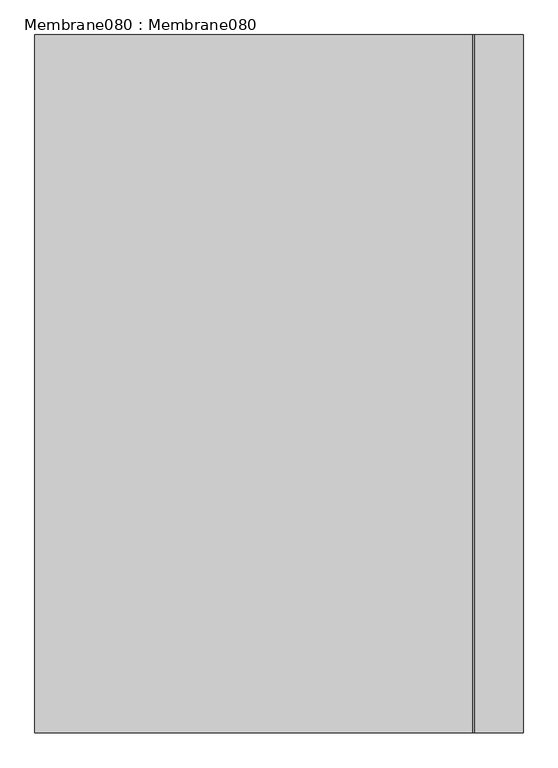
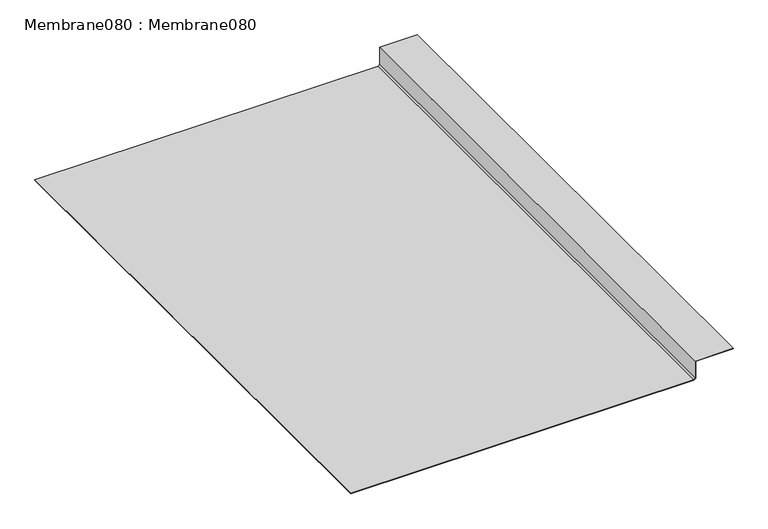
"""IFC4 building model written with IfcOpenShell, lengths in millimetres: proxy geometry, Membrane080 : Membrane080."""

from ifc_helpers import new_model, si_unit, frame, origin, place, context, project, spatial, polyline, outline, extrude, source, transform, mapped, element, save


def membrane080_membrane080_50d92a24(model_context):
    return source(origin(), model_context, "Body", "SweptSolid", [
        extrude(outline(polyline([(36549.109375, -1995.5294189), (36549.109375, -2134.3322754), (36483.4346119, -2134.3322754), (36478.390625, -2139.6929064), (36478.390625, -3395.3427853), (36476.390625, -3395.3427853), (36476.390625, -2138.8999023), (36482.5703125, -2132.3322754), (36547.109375, -2132.3322754), (36547.109375, -1995.5294189), (36549.109375, -1995.5294189)])), frame((0.0, 998.1570053, 0.0), z_axis=(0.0, 1.0, 0.0), x_axis=(0.0, 0.0, 1.0)), (0.0, 0.0, 1.0), 2000.0),
    ])


if __name__ == "__main__":
    model = new_model("IFC4")
    model_context = context("Model", 3, world=origin())
    ifc_project = project(units=[si_unit("LENGTHUNIT", "METRE", prefix="MILLI")], contexts=[model_context])
    site = spatial("IfcSite", under=ifc_project)
    building = spatial("IfcBuilding", under=site)
    placement = place(None, origin())
    membrane080_membrane080_shape = membrane080_membrane080_50d92a24(model_context)
    element("IfcBuildingElementProxy", 1, Name="Membrane080 : Membrane080", ObjectType="Membrane080 : Membrane080", at=placement, inside=building, context=model_context, shape_type="MappedRepresentation", body=[
        mapped(membrane080_membrane080_shape, transform((0.0, 0.0, 0.0), x_axis=(1.0, 0.0, 0.0), y_axis=(0.0, 1.0, 0.0), z_axis=(0.0, 0.0, 1.0))),
    ])
    save(model, "model.ifc")

# Revit data of these elements
# Type "Membrane080 : Membrane080"
#   NameOverride = "Membrane080"
# Element 1 (IfcBuildingElementProxy, "Membrane080 : Membrane080")
#   Materials on its faces: "WESTCOAT ALX UNDER TILE WATERPROOFING SYSTEM (FOLLOW MANUFACTURER'S INSTALLATION REQUIREMENTS)"
# Materials
#   "WESTCOAT ALX UNDER TILE WATERPROOFING SYSTEM (FOLLOW MANUFACTURER'S INSTALLATION REQUIREMENTS)": class "Unassigned", colour RGB 179 255 168, transparency 0, Cost = 0
